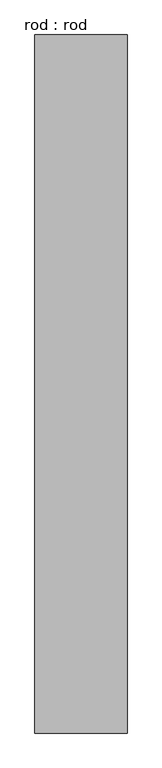
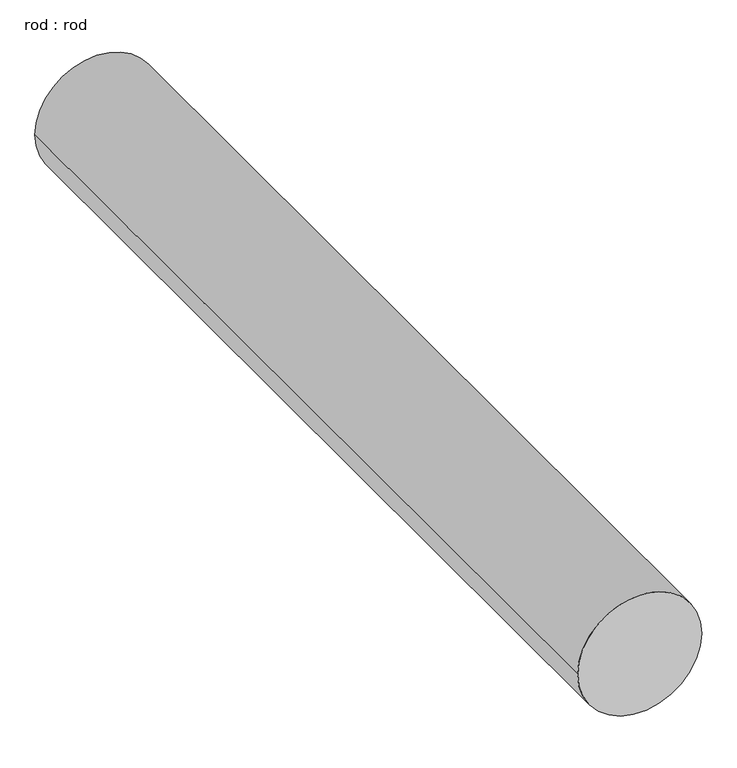
"""IFC4 building model written with IfcOpenShell, lengths in millimetres: proxy geometry, rod : rod."""

import ifcopenshell
import ifcopenshell.guid

model = None  # the IFC model being written
_history = None  # IfcOwnerHistory: only IFC2X3 demands one
_inside = {}  # id of a spatial element -> (the spatial element, [elements in it])
_under = {}  # id of a project, library or spatial element -> (it, [spatial elements below it])
_declared = {}  # id of a project -> (the project, [libraries it declares])
_typed = {}  # id of a type object -> (the type object, [elements of that type])
_made_of = {}  # id of a material, layer set ... -> (it, [elements and type objects made of it])


def new_model(schema):
    """Start an empty IFC model of exactly this schema.

    Asked for "IFC4X3", IfcOpenShell would pick the latest addendum, in which some entities
    have other attributes; the version numbers below select the first issue.
    IFC2X3 requires an IfcOwnerHistory on every rooted entity: one is made here for all.
    """
    global model, _history
    if schema == "IFC4X3":
        model = ifcopenshell.file(schema_version=(4, 3, 0, 0))
    else:
        model = ifcopenshell.file(schema=schema)
    _inside.clear()
    _under.clear()
    _declared.clear()
    _typed.clear()
    _made_of.clear()
    _history = None
    if model.schema == "IFC2X3":
        org = make("IfcOrganization", Name="unknown")
        user = make(
            "IfcPersonAndOrganization",
            ThePerson=make("IfcPerson", FamilyName="unknown"),
            TheOrganization=org,
        )
        app = make(
            "IfcApplication",
            ApplicationDeveloper=org,
            Version="unknown",
            ApplicationFullName="unknown",
            ApplicationIdentifier="unknown",
        )
        _history = make(
            "IfcOwnerHistory",
            OwningUser=user,
            OwningApplication=app,
            ChangeAction="ADDED",
            CreationDate=0,
        )
    return model


def make(cls, **values):
    """One entity of the class cls with the attributes given. An attribute that is None is left unset."""
    return model.create_entity(
        cls, **{name: value for name, value in values.items() if value is not None}
    )


def rooted(cls, **values):
    """An entity with a GlobalId (a new one), such as an element, a storey or a relation."""
    return make(cls, GlobalId=ifcopenshell.guid.new(), OwnerHistory=_history, **values)


def si_unit(unit_type, name, prefix=None):
    """IfcSIUnit, for example si_unit("LENGTHUNIT", "METRE", prefix="MILLI")."""
    return make("IfcSIUnit", UnitType=unit_type, Prefix=prefix, Name=name)


def assignment(units):
    """IfcUnitAssignment: the units of a project."""
    return None if units is None else make("IfcUnitAssignment", Units=units)


def point(xyz):
    """IfcCartesianPoint."""
    return None if xyz is None else make("IfcCartesianPoint", Coordinates=xyz)


def direction(xyz):
    """IfcDirection."""
    return None if xyz is None else make("IfcDirection", DirectionRatios=xyz)


def frame(location, z_axis=None, x_axis=None):
    """IfcAxis2Placement3D, a coordinate frame: its origin and axes. An axis left out is left unset."""
    return make(
        "IfcAxis2Placement3D",
        Location=point(location),
        Axis=direction(z_axis),
        RefDirection=direction(x_axis),
    )


def frame_2d(location, x_axis=None):
    """IfcAxis2Placement2D, a coordinate frame in the plane: its origin and x axis."""
    return make(
        "IfcAxis2Placement2D", Location=point(location), RefDirection=direction(x_axis)
    )


def origin():
    """The frame at (0, 0, 0) with its axes left unset."""
    return frame((0.0, 0.0, 0.0))


def place(relative_to, where):
    """IfcLocalPlacement: puts the frame where relative to a parent placement (None: the world)."""
    return make(
        "IfcLocalPlacement", PlacementRelTo=relative_to, RelativePlacement=where
    )


def context(
    kind, dimensions, precision=None, world=None, true_north=None, identifier=None
):
    """IfcGeometricRepresentationContext, for example the 3D "Model" context."""
    return make(
        "IfcGeometricRepresentationContext",
        ContextIdentifier=identifier,
        ContextType=kind,
        CoordinateSpaceDimension=dimensions,
        Precision=precision,
        WorldCoordinateSystem=world,
        TrueNorth=true_north,
    )


def project(units=None, contexts=None):
    """IfcProject with its units and contexts."""
    return rooted(
        "IfcProject",
        Name="project",
        RepresentationContexts=contexts,
        UnitsInContext=assignment(units),
    )


def spatial(cls, under=None, at=None, **own):
    """A site, building, storey or space (cls), placed at a placement, below another one or the project."""
    s = rooted(cls, ObjectPlacement=at, **own)
    if under is not None:
        _under.setdefault(under.id(), (under, []))[1].append(s)
    return s


def circle_curve(where, radius):
    """IfcCircle in the frame where."""
    return make("IfcCircle", Position=where, Radius=radius)


def trimmed(basis, trim1, trim2, sense, master):
    """IfcTrimmedCurve: the piece of a basis curve between two trims."""
    return make(
        "IfcTrimmedCurve",
        BasisCurve=basis,
        Trim1=trim1,
        Trim2=trim2,
        SenseAgreement=sense,
        MasterRepresentation=master,
    )


def segment(curve, same_sense, transition):
    """IfcCompositeCurveSegment."""
    return make(
        "IfcCompositeCurveSegment",
        Transition=transition,
        SameSense=same_sense,
        ParentCurve=curve,
    )


def composite_curve(segments, self_intersect=None):
    """IfcCompositeCurve: segments joined end to end."""
    return make("IfcCompositeCurve", Segments=segments, SelfIntersect=self_intersect)


def outline(outer, holes=None, kind="AREA"):
    """IfcArbitraryClosedProfileDef: a profile drawn as a closed curve; with holes, ...WithVoids."""
    if holes is None:
        return make("IfcArbitraryClosedProfileDef", ProfileType=kind, OuterCurve=outer)
    return make(
        "IfcArbitraryProfileDefWithVoids",
        ProfileType=kind,
        OuterCurve=outer,
        InnerCurves=holes,
    )


def extrude(swept, where, along, depth):
    """IfcExtrudedAreaSolid: the profile swept, set in the frame where, extruded along a direction by depth."""
    return make(
        "IfcExtrudedAreaSolid",
        SweptArea=swept,
        Position=where,
        ExtrudedDirection=direction(along),
        Depth=depth,
    )


def shape(context_of_items, identifier, shape_type, items):
    """IfcShapeRepresentation: the items that make up one representation, for example the "Body"."""
    return make(
        "IfcShapeRepresentation",
        ContextOfItems=context_of_items,
        RepresentationIdentifier=identifier,
        RepresentationType=shape_type,
        Items=items,
    )


def source(mapping_origin, context_of_items, identifier, shape_type, items):
    """IfcRepresentationMap: a shape defined once, which mapped items show again and again."""
    return make(
        "IfcRepresentationMap",
        MappingOrigin=mapping_origin,
        MappedRepresentation=shape(context_of_items, identifier, shape_type, items),
    )


def transform(
    local_origin,
    x_axis=None,
    y_axis=None,
    z_axis=None,
    scale=None,
    scale2=None,
    scale3=None,
    uniform=True,
):
    """IfcCartesianTransformationOperator3D, or its non-uniform kind. x_axis, y_axis, z_axis: its Axis1, 2, 3."""
    if uniform:
        return make(
            "IfcCartesianTransformationOperator3D",
            Axis1=direction(x_axis),
            Axis2=direction(y_axis),
            LocalOrigin=point(local_origin),
            Scale=scale,
            Axis3=direction(z_axis),
        )
    return make(
        "IfcCartesianTransformationOperator3DnonUniform",
        Axis1=direction(x_axis),
        Axis2=direction(y_axis),
        LocalOrigin=point(local_origin),
        Scale=scale,
        Axis3=direction(z_axis),
        Scale2=scale2,
        Scale3=scale3,
    )


def mapped(mapping_source, mapping_target):
    """IfcMappedItem: shows the shape of a source again, moved by a transform."""
    return make(
        "IfcMappedItem", MappingSource=mapping_source, MappingTarget=mapping_target
    )


def made_of(thing, what):
    """Note that an element or type object is made of a material, layer set ...; save() writes the relation."""
    if what is not None:
        _made_of.setdefault(what.id(), (what, []))[1].append(thing)
    return thing


def element(
    cls,
    number,
    at=None,
    inside=None,
    cuts=None,
    type_object=None,
    material=None,
    context=None,
    identifier="Body",
    shape_type=None,
    held_by="IfcProductDefinitionShape",
    body=None,
    shapes=None,
    **own,
):
    """One element of the class cls, such as IfcWall. Its Tag is "e" and its number.

    at: its placement. inside: the storey or other place that contains it. cuts: it is an
    opening in that element (IfcRelVoidsElement). A single representation is given by context,
    identifier, shape_type and body (its items); several are given by shapes. held_by: the class
    of the entity that holds the representations. save() writes the other relations.
    """
    e = rooted(cls, Tag="e%d" % number, ObjectPlacement=at, **own)
    if body is not None:
        shapes = [shape(context, identifier, shape_type, body)]
    if shapes is not None:
        e.Representation = make(held_by, Representations=shapes)
    if inside is not None:
        _inside.setdefault(inside.id(), (inside, []))[1].append(e)
    if cuts is not None:
        rooted(
            "IfcRelVoidsElement", RelatingBuildingElement=cuts, RelatedOpeningElement=e
        )
    if type_object is not None:
        _typed.setdefault(type_object.id(), (type_object, []))[1].append(e)
    return made_of(e, material)


def aggregate(whole, parts):
    """IfcRelAggregates: a whole, such as a stair, and the parts it consists of."""
    return rooted("IfcRelAggregates", RelatingObject=whole, RelatedObjects=parts)


def save(model, path):
    """Write the relations noted so far, then the file.

    IfcRelAggregates (storeys below a building ...), IfcRelContainedInSpatialStructure (elements
    in a storey), IfcRelDefinesByType, IfcRelAssociatesMaterial and IfcRelDeclares: one each for
    every whole, place, type object, material and project.
    """
    for whole, parts in _under.values():
        aggregate(whole, parts)
    for where, things in _inside.values():
        rooted(
            "IfcRelContainedInSpatialStructure",
            RelatedElements=things,
            RelatingStructure=where,
        )
    for kind, things in _typed.values():
        rooted("IfcRelDefinesByType", RelatedObjects=things, RelatingType=kind)
    for what, things in _made_of.values():
        rooted("IfcRelAssociatesMaterial", RelatedObjects=things, RelatingMaterial=what)
    for by, libraries in _declared.values():
        rooted("IfcRelDeclares", RelatingContext=by, RelatedDefinitions=libraries)
    model.write(path)


def rod_rod_f3586d77(model_context):
    return source(origin(), model_context, "Body", "SweptSolid", [
        extrude(outline(composite_curve([segment(trimmed(circle_curve(frame_2d((0.0108462, 0.0)), 200.0), [point((0.0108462, 200.0))], [point((0.0108462, -200.0))], False, "CARTESIAN"), True, "CONTINUOUS"), segment(trimmed(circle_curve(frame_2d((0.0108462, 0.0)), 200.0), [point((0.0108462, -200.0))], [point((0.0108462, 200.0))], False, "CARTESIAN"), True, "CONTINUOUS")], self_intersect=False)), frame((0.0, 2576.6571868, 0.0), z_axis=(0.0, 1.0, 0.0), x_axis=(0.0, 0.0, 1.0)), (0.0, 0.0, 1.0), 3032.1428571),
    ])


if __name__ == "__main__":
    model = new_model("IFC4")
    model_context = context("Model", 3, world=origin())
    ifc_project = project(units=[si_unit("LENGTHUNIT", "METRE", prefix="MILLI")], contexts=[model_context])
    site = spatial("IfcSite", under=ifc_project)
    building = spatial("IfcBuilding", under=site)
    placement = place(None, origin())
    rod_rod_shape = rod_rod_f3586d77(model_context)
    element("IfcBuildingElementProxy", 1, Name="rod : rod", ObjectType="rod : rod", at=placement, inside=building, context=model_context, shape_type="MappedRepresentation", body=[
        mapped(rod_rod_shape, transform((0.0, 0.0, 0.0), x_axis=(1.0, 0.0, 0.0), y_axis=(0.0, 1.0, 0.0), z_axis=(0.0, 0.0, 1.0))),
    ])
    save(model, "model.ifc")

# Revit data of these elements
# Type "rod : rod"
#   Default Elevation = 0
